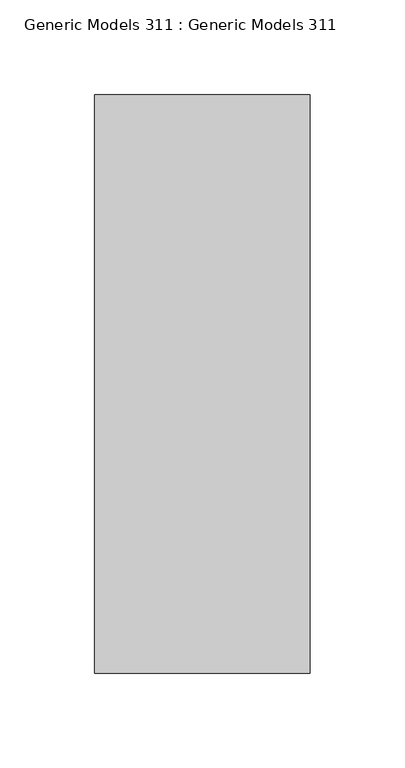
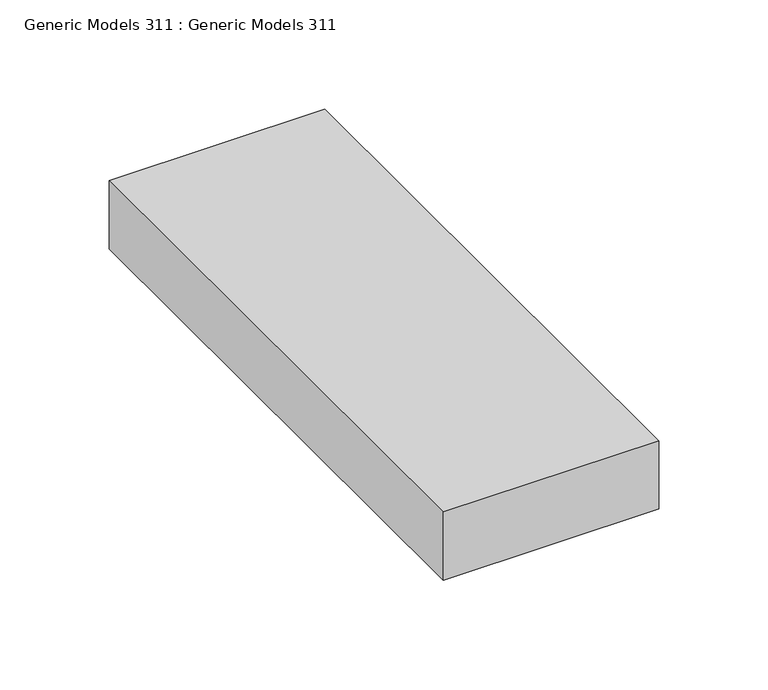
"""IFC4 building model written with IfcOpenShell, lengths in millimetres: proxy geometry, Generic Models 311 : Generic Models 311."""

from ifc_helpers import new_model, si_unit, frame, origin, place, context, project, spatial, polyline, outline, extrude, source, transform, mapped, element, save


def generic_models_311_generic_models_311_135e98dc(model_context):
    return source(origin(), model_context, "Body", "SweptSolid", [
        extrude(outline(polyline([(3531.1804357, 704.5309662), (3644.7263704, 704.5309662), (3644.7263704, 399.7309662), (3531.1804357, 399.7309662), (3531.1804357, 704.5309662)])), frame((0.0, 0.0, 124415.9105709), z_axis=(0.0, 0.0, 1.0), x_axis=(1.0, 0.0, 0.0)), (0.0, 0.0, 1.0), 38.1),
    ])


if __name__ == "__main__":
    model = new_model("IFC4")
    model_context = context("Model", 3, world=origin())
    ifc_project = project(units=[si_unit("LENGTHUNIT", "METRE", prefix="MILLI")], contexts=[model_context])
    site = spatial("IfcSite", under=ifc_project)
    building = spatial("IfcBuilding", under=site)
    placement = place(None, origin())
    generic_models_311_generic_models_311_shape = generic_models_311_generic_models_311_135e98dc(model_context)
    element("IfcBuildingElementProxy", 1, Name="Generic Models 311 : Generic Models 311", ObjectType="Generic Models 311 : Generic Models 311", at=placement, inside=building, context=model_context, shape_type="MappedRepresentation", body=[
        mapped(generic_models_311_generic_models_311_shape, transform((0.0, 0.0, 0.0), x_axis=(1.0, 0.0, 0.0), y_axis=(0.0, 1.0, 0.0), z_axis=(0.0, 0.0, 1.0))),
    ])
    save(model, "model.ifc")

# Revit data of these elements
# Element 1 (IfcBuildingElementProxy, "Generic Models 311 : Generic Models 311")
#   Materials on its faces: "_BLOCKING AS REQUIRED"
# Materials
#   "_BLOCKING AS REQUIRED": class "Generic", colour RGB 177 130 114, transparency 0, Cost = 0
